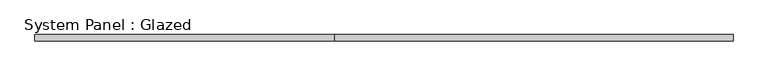
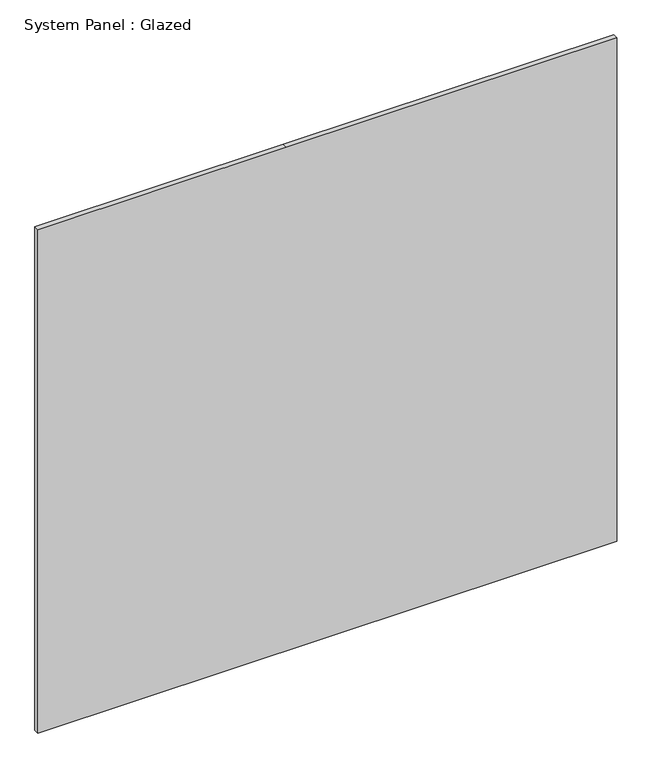
"""IFC4 building model written with IfcOpenShell, lengths in millimetres: plate geometry, System Panel : Glazed."""

from ifc_helpers import new_model, si_unit, frame, origin, place, context, project, spatial, polyline, outline, extrude, source, transform, mapped, element, save


def system_panel_glazed_8c6f7263(model_context):
    return source(origin(), model_context, "Body", "SweptSolid", [
        extrude(outline(polyline([(0.0, -2767.2293345), (0.0, 2767.2293345), (5090.0, 2767.2293345), (5090.0, -390.5342272), (5090.0, -2767.2293345), (0.0, -2767.2293345)])), frame((0.0, -25.0, 0.0), z_axis=(0.0, 1.0, 0.0), x_axis=(0.0, 0.0, 1.0)), (0.0, 0.0, 1.0), 50.0),
    ])


if __name__ == "__main__":
    model = new_model("IFC4")
    model_context = context("Model", 3, world=origin())
    ifc_project = project(units=[si_unit("LENGTHUNIT", "METRE", prefix="MILLI")], contexts=[model_context])
    site = spatial("IfcSite", under=ifc_project)
    building = spatial("IfcBuilding", under=site)
    placement = place(None, origin())
    system_panel_glazed_shape = system_panel_glazed_8c6f7263(model_context)
    element("IfcPlate", 1, ObjectType="System Panel : Glazed", at=placement, inside=building, context=model_context, shape_type="MappedRepresentation", body=[
        mapped(system_panel_glazed_shape, transform((0.0, 0.0, 0.0), x_axis=(1.0, 0.0, 0.0), y_axis=(0.0, 1.0, 0.0), z_axis=(0.0, 0.0, 1.0))),
    ])
    save(model, "model.ifc")

# Revit data of these elements
# Type "System Panel : Glazed"
#   Type Mark = "CW-GLASS"
# Element 1 (IfcPlate, "System Panel : Glazed")
#   Materials on its faces: "Glass_Clear"
# Materials
#   "Glass_Clear": class "Glass", colour RGB 128 128 255, transparency 0.8, Comments = "Rendering appearance not upgraded ", Cost = 0
